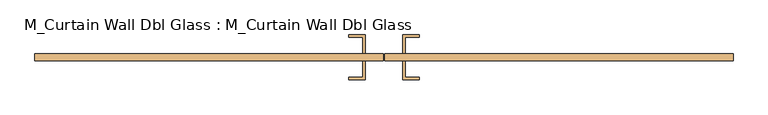
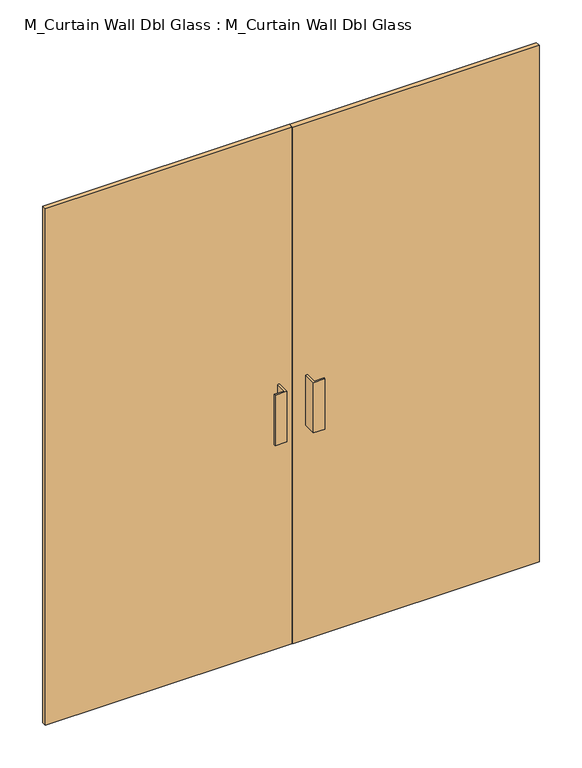
"""IFC4 building model written with IfcOpenShell, lengths in millimetres: door geometry, M_Curtain Wall Dbl Glass : M_Curtain Wall Dbl Glass."""

from ifc_helpers import new_model, si_unit, frame, origin, origin_with_axes, place, context, project, spatial, polyline, outline, extrude, source, transform, mapped, element, save


def m_curtain_wall_dbl_glass_m_curtain_wall_dbl_glass_49306077(model_context):
    return source(origin(), model_context, "Body", "SweptSolid", [
        extrude(outline(polyline([(-1.5875, -30.95), (-1.5875, -50.0), (-942.5, -50.0), (-942.5, -30.95), (-1.5875, -30.95)])), origin_with_axes(), (0.0, 0.0, 1.0), 2085.0),
        extrude(outline(polyline([(942.5, -30.95), (942.5, -50.0), (1.5875, -50.0), (1.5875, -30.95), (942.5, -30.95)])), origin_with_axes(), (0.0, 0.0, 1.0), 2085.0),
        extrude(outline(polyline([(-50.8, -100.8), (-95.25, -100.8), (-95.25, -94.45), (-57.15, -94.45), (-57.15, -50.0), (-50.8, -50.0), (-50.8, -100.8)])), frame((0.0, 0.0, 863.6), z_axis=(0.0, 0.0, 1.0), x_axis=(1.0, 0.0, 0.0)), (0.0, 0.0, 1.0), 203.2),
        extrude(outline(polyline([(50.8, -100.8), (50.8, -50.0), (57.15, -50.0), (57.15, -94.45), (95.25, -94.45), (95.25, -100.8), (50.8, -100.8)])), frame((0.0, 0.0, 863.6), z_axis=(0.0, 0.0, 1.0), x_axis=(1.0, 0.0, 0.0)), (0.0, 0.0, 1.0), 203.2),
        extrude(outline(polyline([(-50.8, 19.85), (-50.8, -30.95), (-57.15, -30.95), (-57.15, 13.5), (-95.25, 13.5), (-95.25, 19.85), (-50.8, 19.85)])), frame((0.0, 0.0, 863.6), z_axis=(0.0, 0.0, 1.0), x_axis=(1.0, 0.0, 0.0)), (0.0, 0.0, 1.0), 203.2),
        extrude(outline(polyline([(50.8, 19.85), (95.25, 19.85), (95.25, 13.5), (57.15, 13.5), (57.15, -30.95), (50.8, -30.95), (50.8, 19.85)])), frame((0.0, 0.0, 863.6), z_axis=(0.0, 0.0, 1.0), x_axis=(1.0, 0.0, 0.0)), (0.0, 0.0, 1.0), 203.2),
    ])


if __name__ == "__main__":
    model = new_model("IFC4")
    model_context = context("Model", 3, world=origin())
    ifc_project = project(units=[si_unit("LENGTHUNIT", "METRE", prefix="MILLI")], contexts=[model_context])
    site = spatial("IfcSite", under=ifc_project)
    building = spatial("IfcBuilding", under=site)
    placement = place(None, origin())
    m_curtain_wall_dbl_glass_m_curtain_wall_dbl_glass_shape = m_curtain_wall_dbl_glass_m_curtain_wall_dbl_glass_49306077(model_context)
    element("IfcDoor", 1, ObjectType="M_Curtain Wall Dbl Glass : M_Curtain Wall Dbl Glass", at=placement, inside=building, context=model_context, shape_type="MappedRepresentation", body=[
        mapped(m_curtain_wall_dbl_glass_m_curtain_wall_dbl_glass_shape, transform((0.0, 0.0, 0.0), x_axis=(1.0, 0.0, 0.0), y_axis=(0.0, 1.0, 0.0), z_axis=(0.0, 0.0, 1.0))),
    ])
    save(model, "model.ifc")

# Revit data of these elements
# Type "M_Curtain Wall Dbl Glass : M_Curtain Wall Dbl Glass"
#   Model = "12345678"
#   Manufacturer = "Dublin Doors"
#   Description = "Double Glass Door"
#   Type Mark = "41"
#   COBie.Type.CreatedBy = "design@eagle.com"
#   COBie.Type.CreatedOn = "2016-09-13T05:47:35"
#   COBie.Type.Name = "Doors_M_Curtain Wall Dbl Glass_M_Curtain Wall Dbl Glass"
#   COBie.Type.Category = "23-30 10 00 : Doors"
#   COBie.Type.Description = "Double Glass Door"
#   COBie.Type.Manufacturer = "Dublin Doors"
#   COBie.Type.ModelNumber = "12345678"
#   Construction Type Id = "GSP4R"
#   Analytic Construction = "1/8 in Pilkington single glazing"
#   COBie.Type.ReplacementCost = 0
#   Visual Light Transmittance = 0.9
#   Solar Heat Gain Coefficient = 0.78
#   Offset = 50 mm
#   Heat Transfer Coefficient (U) = 3.6886 W/(m²·K)
#   COBie.Type = yes
#   Function = 1
#   Glazing Material = Glass
# Element 1 (IfcDoor, "M_Curtain Wall Dbl Glass : M_Curtain Wall Dbl Glass")
#   Materials on its faces: "Aluminum", "Glass"
# Materials
#   "Glass": class "Glass", colour RGB 0 128 192, transparency 0.75, Description = "Soda Lime Glass", Cost = 0
#   "Aluminum": class "Metal", colour RGB 247 247 247, transparency 0, Description = "Aluminum 6061", Cost = 0
